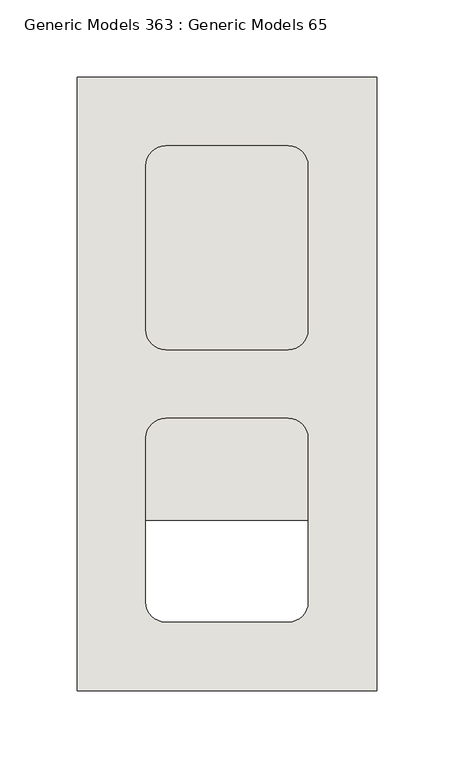
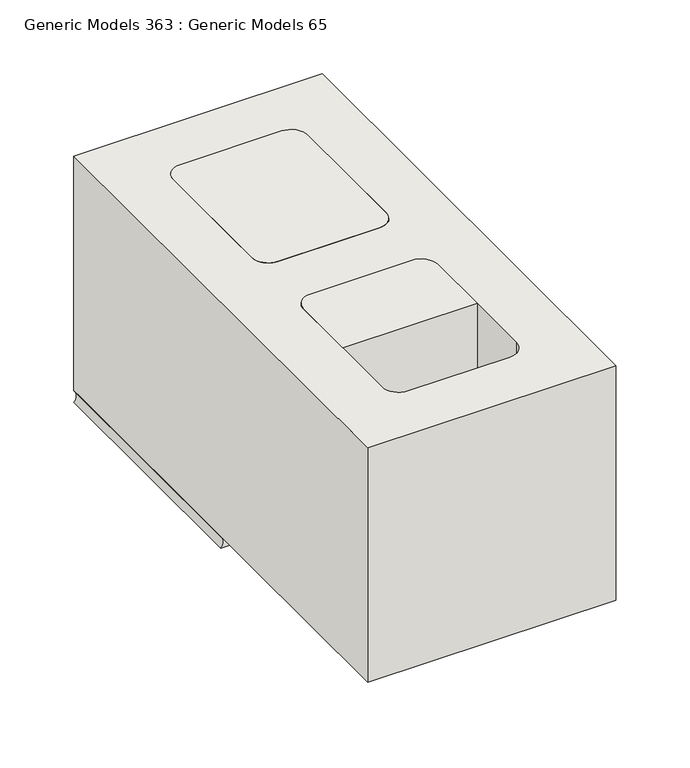
"""IFC4 building model written with IfcOpenShell, lengths in millimetres: wall geometry, Generic Models 363 : Generic Models 65."""

import ifcopenshell
import ifcopenshell.guid

model = None  # the IFC model being written
_history = None  # IfcOwnerHistory: only IFC2X3 demands one
_inside = {}  # id of a spatial element -> (the spatial element, [elements in it])
_under = {}  # id of a project, library or spatial element -> (it, [spatial elements below it])
_declared = {}  # id of a project -> (the project, [libraries it declares])
_typed = {}  # id of a type object -> (the type object, [elements of that type])
_made_of = {}  # id of a material, layer set ... -> (it, [elements and type objects made of it])


def new_model(schema):
    """Start an empty IFC model of exactly this schema.

    Asked for "IFC4X3", IfcOpenShell would pick the latest addendum, in which some entities
    have other attributes; the version numbers below select the first issue.
    IFC2X3 requires an IfcOwnerHistory on every rooted entity: one is made here for all.
    """
    global model, _history
    if schema == "IFC4X3":
        model = ifcopenshell.file(schema_version=(4, 3, 0, 0))
    else:
        model = ifcopenshell.file(schema=schema)
    _inside.clear()
    _under.clear()
    _declared.clear()
    _typed.clear()
    _made_of.clear()
    _history = None
    if model.schema == "IFC2X3":
        org = make("IfcOrganization", Name="unknown")
        user = make(
            "IfcPersonAndOrganization",
            ThePerson=make("IfcPerson", FamilyName="unknown"),
            TheOrganization=org,
        )
        app = make(
            "IfcApplication",
            ApplicationDeveloper=org,
            Version="unknown",
            ApplicationFullName="unknown",
            ApplicationIdentifier="unknown",
        )
        _history = make(
            "IfcOwnerHistory",
            OwningUser=user,
            OwningApplication=app,
            ChangeAction="ADDED",
            CreationDate=0,
        )
    return model


def make(cls, **values):
    """One entity of the class cls with the attributes given. An attribute that is None is left unset."""
    return model.create_entity(
        cls, **{name: value for name, value in values.items() if value is not None}
    )


def rooted(cls, **values):
    """An entity with a GlobalId (a new one), such as an element, a storey or a relation."""
    return make(cls, GlobalId=ifcopenshell.guid.new(), OwnerHistory=_history, **values)


def si_unit(unit_type, name, prefix=None):
    """IfcSIUnit, for example si_unit("LENGTHUNIT", "METRE", prefix="MILLI")."""
    return make("IfcSIUnit", UnitType=unit_type, Prefix=prefix, Name=name)


def assignment(units):
    """IfcUnitAssignment: the units of a project."""
    return None if units is None else make("IfcUnitAssignment", Units=units)


def point(xyz):
    """IfcCartesianPoint."""
    return None if xyz is None else make("IfcCartesianPoint", Coordinates=xyz)


def direction(xyz):
    """IfcDirection."""
    return None if xyz is None else make("IfcDirection", DirectionRatios=xyz)


def frame(location, z_axis=None, x_axis=None):
    """IfcAxis2Placement3D, a coordinate frame: its origin and axes. An axis left out is left unset."""
    return make(
        "IfcAxis2Placement3D",
        Location=point(location),
        Axis=direction(z_axis),
        RefDirection=direction(x_axis),
    )


def frame_2d(location, x_axis=None):
    """IfcAxis2Placement2D, a coordinate frame in the plane: its origin and x axis."""
    return make(
        "IfcAxis2Placement2D", Location=point(location), RefDirection=direction(x_axis)
    )


def origin():
    """The frame at (0, 0, 0) with its axes left unset."""
    return frame((0.0, 0.0, 0.0))


def place(relative_to, where):
    """IfcLocalPlacement: puts the frame where relative to a parent placement (None: the world)."""
    return make(
        "IfcLocalPlacement", PlacementRelTo=relative_to, RelativePlacement=where
    )


def context(
    kind, dimensions, precision=None, world=None, true_north=None, identifier=None
):
    """IfcGeometricRepresentationContext, for example the 3D "Model" context."""
    return make(
        "IfcGeometricRepresentationContext",
        ContextIdentifier=identifier,
        ContextType=kind,
        CoordinateSpaceDimension=dimensions,
        Precision=precision,
        WorldCoordinateSystem=world,
        TrueNorth=true_north,
    )


def project(units=None, contexts=None):
    """IfcProject with its units and contexts."""
    return rooted(
        "IfcProject",
        Name="project",
        RepresentationContexts=contexts,
        UnitsInContext=assignment(units),
    )


def spatial(cls, under=None, at=None, **own):
    """A site, building, storey or space (cls), placed at a placement, below another one or the project."""
    s = rooted(cls, ObjectPlacement=at, **own)
    if under is not None:
        _under.setdefault(under.id(), (under, []))[1].append(s)
    return s


def polyline(points):
    """IfcPolyline through the points."""
    return make("IfcPolyline", Points=[point(p) for p in points])


def circle_curve(where, radius):
    """IfcCircle in the frame where."""
    return make("IfcCircle", Position=where, Radius=radius)


def trimmed(basis, trim1, trim2, sense, master):
    """IfcTrimmedCurve: the piece of a basis curve between two trims."""
    return make(
        "IfcTrimmedCurve",
        BasisCurve=basis,
        Trim1=trim1,
        Trim2=trim2,
        SenseAgreement=sense,
        MasterRepresentation=master,
    )


def segment(curve, same_sense, transition):
    """IfcCompositeCurveSegment."""
    return make(
        "IfcCompositeCurveSegment",
        Transition=transition,
        SameSense=same_sense,
        ParentCurve=curve,
    )


def composite_curve(segments, self_intersect=None):
    """IfcCompositeCurve: segments joined end to end."""
    return make("IfcCompositeCurve", Segments=segments, SelfIntersect=self_intersect)


def outline(outer, holes=None, kind="AREA"):
    """IfcArbitraryClosedProfileDef: a profile drawn as a closed curve; with holes, ...WithVoids."""
    if holes is None:
        return make("IfcArbitraryClosedProfileDef", ProfileType=kind, OuterCurve=outer)
    return make(
        "IfcArbitraryProfileDefWithVoids",
        ProfileType=kind,
        OuterCurve=outer,
        InnerCurves=holes,
    )


def extrude(swept, where, along, depth):
    """IfcExtrudedAreaSolid: the profile swept, set in the frame where, extruded along a direction by depth."""
    return make(
        "IfcExtrudedAreaSolid",
        SweptArea=swept,
        Position=where,
        ExtrudedDirection=direction(along),
        Depth=depth,
    )


def shape(context_of_items, identifier, shape_type, items):
    """IfcShapeRepresentation: the items that make up one representation, for example the "Body"."""
    return make(
        "IfcShapeRepresentation",
        ContextOfItems=context_of_items,
        RepresentationIdentifier=identifier,
        RepresentationType=shape_type,
        Items=items,
    )


def source(mapping_origin, context_of_items, identifier, shape_type, items):
    """IfcRepresentationMap: a shape defined once, which mapped items show again and again."""
    return make(
        "IfcRepresentationMap",
        MappingOrigin=mapping_origin,
        MappedRepresentation=shape(context_of_items, identifier, shape_type, items),
    )


def transform(
    local_origin,
    x_axis=None,
    y_axis=None,
    z_axis=None,
    scale=None,
    scale2=None,
    scale3=None,
    uniform=True,
):
    """IfcCartesianTransformationOperator3D, or its non-uniform kind. x_axis, y_axis, z_axis: its Axis1, 2, 3."""
    if uniform:
        return make(
            "IfcCartesianTransformationOperator3D",
            Axis1=direction(x_axis),
            Axis2=direction(y_axis),
            LocalOrigin=point(local_origin),
            Scale=scale,
            Axis3=direction(z_axis),
        )
    return make(
        "IfcCartesianTransformationOperator3DnonUniform",
        Axis1=direction(x_axis),
        Axis2=direction(y_axis),
        LocalOrigin=point(local_origin),
        Scale=scale,
        Axis3=direction(z_axis),
        Scale2=scale2,
        Scale3=scale3,
    )


def mapped(mapping_source, mapping_target):
    """IfcMappedItem: shows the shape of a source again, moved by a transform."""
    return make(
        "IfcMappedItem", MappingSource=mapping_source, MappingTarget=mapping_target
    )


def made_of(thing, what):
    """Note that an element or type object is made of a material, layer set ...; save() writes the relation."""
    if what is not None:
        _made_of.setdefault(what.id(), (what, []))[1].append(thing)
    return thing


def element(
    cls,
    number,
    at=None,
    inside=None,
    cuts=None,
    type_object=None,
    material=None,
    context=None,
    identifier="Body",
    shape_type=None,
    held_by="IfcProductDefinitionShape",
    body=None,
    shapes=None,
    **own,
):
    """One element of the class cls, such as IfcWall. Its Tag is "e" and its number.

    at: its placement. inside: the storey or other place that contains it. cuts: it is an
    opening in that element (IfcRelVoidsElement). A single representation is given by context,
    identifier, shape_type and body (its items); several are given by shapes. held_by: the class
    of the entity that holds the representations. save() writes the other relations.
    """
    e = rooted(cls, Tag="e%d" % number, ObjectPlacement=at, **own)
    if body is not None:
        shapes = [shape(context, identifier, shape_type, body)]
    if shapes is not None:
        e.Representation = make(held_by, Representations=shapes)
    if inside is not None:
        _inside.setdefault(inside.id(), (inside, []))[1].append(e)
    if cuts is not None:
        rooted(
            "IfcRelVoidsElement", RelatingBuildingElement=cuts, RelatedOpeningElement=e
        )
    if type_object is not None:
        _typed.setdefault(type_object.id(), (type_object, []))[1].append(e)
    return made_of(e, material)


def aggregate(whole, parts):
    """IfcRelAggregates: a whole, such as a stair, and the parts it consists of."""
    return rooted("IfcRelAggregates", RelatingObject=whole, RelatedObjects=parts)


def save(model, path):
    """Write the relations noted so far, then the file.

    IfcRelAggregates (storeys below a building ...), IfcRelContainedInSpatialStructure (elements
    in a storey), IfcRelDefinesByType, IfcRelAssociatesMaterial and IfcRelDeclares: one each for
    every whole, place, type object, material and project.
    """
    for whole, parts in _under.values():
        aggregate(whole, parts)
    for where, things in _inside.values():
        rooted(
            "IfcRelContainedInSpatialStructure",
            RelatedElements=things,
            RelatingStructure=where,
        )
    for kind, things in _typed.values():
        rooted("IfcRelDefinesByType", RelatedObjects=things, RelatingType=kind)
    for what, things in _made_of.values():
        rooted("IfcRelAssociatesMaterial", RelatedObjects=things, RelatingMaterial=what)
    for by, libraries in _declared.values():
        rooted("IfcRelDeclares", RelatingContext=by, RelatedDefinitions=libraries)
    model.write(path)


def plane_surface(at):
    """IfcPlane: the flat surface through the origin of the frame at, square to its z axis."""
    return make("IfcPlane", Position=at)


def revolved_surface(curve, axis_point, axis_direction):
    """IfcSurfaceOfRevolution: the curve turned about the line through axis_point along axis_direction."""
    return make(
        "IfcSurfaceOfRevolution",
        SweptCurve=make("IfcArbitraryOpenProfileDef", ProfileType="CURVE", Curve=curve),
        AxisPosition=make("IfcAxis1Placement", Location=point(axis_point), Axis=direction(axis_direction)),
    )


def advanced_brep(points, edges, surfaces, faces):
    """IfcAdvancedBrep: a solid bounded by faces that lie on surfaces and meet in shared edges.

    An edge is (start, end): straight between two places in points (the first is 0);
    or (start, end, curve); or (start, end, curve, False) where it runs against its curve.
    A face is (place in surfaces, loops), or (place, loops, False) where it looks against
    its surface's normal. A loop lists edges by number (the first is 1), with a minus sign
    where the edge is run from its end to its start. The first loop is the outer one.
    """
    corners = [point(p) for p in points]
    vertices = [make("IfcVertexPoint", VertexGeometry=c) for c in corners]
    made = []
    for start, end, *more in edges:
        made.append(
            make(
                "IfcEdgeCurve",
                EdgeStart=vertices[start],
                EdgeEnd=vertices[end],
                EdgeGeometry=more[0] if more else make("IfcPolyline", Points=[corners[start], corners[end]]),
                SameSense=more[1] if len(more) > 1 else True,
            )
        )
    hull = []
    for where, loops, *sense in faces:
        bounds = []
        for j, loop in enumerate(loops):
            ring = [make("IfcOrientedEdge", EdgeElement=made[abs(k) - 1], Orientation=k > 0) for k in loop]
            bounds.append(
                make(
                    "IfcFaceOuterBound" if j == 0 else "IfcFaceBound",
                    Bound=make("IfcEdgeLoop", EdgeList=ring),
                    Orientation=True,
                )
            )
        hull.append(make("IfcAdvancedFace", Bounds=bounds, FaceSurface=surfaces[where], SameSense=sense[0] if sense else True))
    return make("IfcAdvancedBrep", Outer=make("IfcClosedShell", CfsFaces=hull))


def generic_models_363_generic_models_65_5e5dd987(model_context):
    return source(origin(), model_context, "Body", "SolidModel", [
        advanced_brep(
        [(430198.2125, 503.2375, 1228.725), (430004.5375, 503.2375, 1228.725), (430004.5375, 503.2375, 1219.2), (430198.2125, 503.2375, 1219.2), (430198.2125, 701.675, 1228.725), (430198.2125, 701.675, 1219.2), (430004.5375, 701.675, 1219.2), (430004.5375, 701.675, 1228.725), (430153.7625, 538.1625, 1228.725), (430141.0625, 525.4625, 1228.725), (430061.6875, 525.4625, 1228.725), (430048.9875, 538.1625, 1228.725), (430048.9875, 644.525, 1228.725), (430061.6875, 657.225, 1228.725), (430141.0625, 657.225, 1228.725), (430153.7625, 644.525, 1228.725), (430141.0625, 525.4625, 1219.2), (430153.7625, 538.1625, 1219.2), (430061.6875, 525.4625, 1219.2), (430048.9875, 538.1625, 1219.2), (430048.9875, 644.525, 1219.2), (430061.6875, 657.225, 1219.2), (430141.0625, 657.225, 1219.2), (430153.7625, 644.525, 1219.2)],
        [
            (0, 1),
            (1, 2, circle_curve(frame((429999.6545028, 503.2375, 1223.9625), z_axis=(0.0, 1.0, 0.0), x_axis=(1.0, 0.0, 0.0)), 6.8209287)),
            (2, 3),
            (3, 0, circle_curve(frame((430203.0954972, 503.2375, 1223.9625), z_axis=(0.0, 1.0, 0.0), x_axis=(-1.0, 0.0, 0.0)), 6.8209287)),
            (4, 5, circle_curve(frame((430203.0954972, 701.675, 1223.9625), z_axis=(0.0, -1.0, 0.0), x_axis=(-1.0, 0.0, 0.0)), 6.8209287)),
            (5, 6),
            (6, 7, circle_curve(frame((429999.6545028, 701.675, 1223.9625), z_axis=(0.0, -1.0, 0.0), x_axis=(1.0, 0.0, 0.0)), 6.8209287)),
            (7, 4),
            (0, 4),
            (7, 1),
            (8, 9, circle_curve(frame((430141.0625, 538.1625, 1228.725), z_axis=(0.0, 0.0, -1.0), x_axis=(-1.0, 0.0, 0.0)), 12.7)),
            (9, 10),
            (10, 11, circle_curve(frame((430061.6875, 538.1625, 1228.725), z_axis=(0.0, 0.0, -1.0), x_axis=(-1.0, 0.0, 0.0)), 12.7)),
            (11, 12),
            (12, 13, circle_curve(frame((430061.6875, 644.525, 1228.725), z_axis=(0.0, 0.0, -1.0), x_axis=(-1.0, 0.0, 0.0)), 12.7)),
            (13, 14),
            (14, 15, circle_curve(frame((430141.0625, 644.525, 1228.725), z_axis=(0.0, 0.0, -1.0), x_axis=(-1.0, 0.0, 0.0)), 12.7)),
            (15, 8),
            (16, 9),
            (8, 17),
            (17, 16, circle_curve(frame((430141.0625, 538.1625, 1219.2), z_axis=(0.0, 0.0, -1.0), x_axis=(-1.0, 0.0, 0.0)), 12.7)),
            (16, 18),
            (18, 10),
            (18, 19, circle_curve(frame((430061.6875, 538.1625, 1219.2), z_axis=(0.0, 0.0, -1.0), x_axis=(-1.0, 0.0, 0.0)), 12.7)),
            (19, 11),
            (19, 20),
            (20, 12),
            (20, 21, circle_curve(frame((430061.6875, 644.525, 1219.2), z_axis=(0.0, 0.0, -1.0), x_axis=(-1.0, 0.0, 0.0)), 12.7)),
            (21, 13),
            (21, 22),
            (22, 14),
            (22, 23, circle_curve(frame((430141.0625, 644.525, 1219.2), z_axis=(0.0, 0.0, -1.0), x_axis=(-1.0, 0.0, 0.0)), 12.7)),
            (23, 15),
            (23, 17),
            (6, 2),
            (5, 3),
        ],
        [
            plane_surface(frame((430101.375, 503.2375, 1229.121875), z_axis=(0.0, -1.0, 0.0), x_axis=(0.0, 0.0, 1.0))),
            plane_surface(frame((430101.375, 701.675, 1229.121875), z_axis=(0.0, 1.0, 0.0), x_axis=(0.0, 0.0, 1.0))),
            plane_surface(frame((430198.2125, 503.2375, 1228.725), z_axis=(0.0, 0.0, 1.0), x_axis=(0.0, 1.0, 0.0))),
            revolved_surface(polyline([(430128.3625, 538.1625, 1228.725), (430128.3625, 538.1625, 1219.2)]), (430141.0625, 538.1625, 1412.875), (0.0, 0.0, 1.0)),
            plane_surface(frame((430061.6875, 525.4625, 1412.875), z_axis=(0.0, 1.0, 0.0), x_axis=(0.0, 0.0, -1.0))),
            revolved_surface(polyline([(430048.9875, 538.1625, 1228.725), (430048.9875, 538.1625, 1219.2)]), (430061.6875, 538.1625, 1412.875), (0.0, 0.0, 1.0)),
            plane_surface(frame((430048.9875, 644.525, 1412.875), z_axis=(1.0, 0.0, 0.0), x_axis=(0.0, 0.0, -1.0))),
            revolved_surface(polyline([(430048.9875, 644.525, 1228.725), (430048.9875, 644.525, 1219.2)]), (430061.6875, 644.525, 1412.875), (0.0, 0.0, 1.0)),
            plane_surface(frame((430141.0625, 657.225, 1412.875), z_axis=(0.0, -1.0, 0.0), x_axis=(0.0, 0.0, -1.0))),
            revolved_surface(polyline([(430128.3625, 644.525, 1228.725), (430128.3625, 644.525, 1219.2)]), (430141.0625, 644.525, 1412.875), (0.0, 0.0, 1.0)),
            plane_surface(frame((430153.7625, 538.1625, 1412.875), z_axis=(-1.0, 0.0, 0.0), x_axis=(0.0, 0.0, -1.0))),
            revolved_surface(polyline([(430006.4754315, 701.675, 1223.9625), (430006.4754315, 503.2375, 1223.9625)]), (429999.6545028, 503.2375, 1223.9625), (0.0, 1.0, 0.0)),
            plane_surface(frame((430004.5375, 503.2375, 1219.2), z_axis=(0.0, 0.0, -1.0), x_axis=(0.0, 1.0, 0.0))),
            revolved_surface(polyline([(430196.2745685, 701.675, 1223.9625), (430196.2745685, 503.2375, 1223.9625)]), (430203.0954972, 503.2375, 1223.9625), (0.0, 1.0, 0.0)),
        ],
        [
            (0, [[1, 2, 3, 4]]),
            (1, [[5, 6, 7, 8]]),
            (2, [[-1, 9, -8, 10], [11, 12, 13, 14, 15, 16, 17, 18]]),
            (3, [[19, -11, 20, 21]]),
            (4, [[-19, 22, 23, -12]]),
            (5, [[-23, 24, 25, -13]]),
            (6, [[-25, 26, 27, -14]]),
            (7, [[-27, 28, 29, -15]]),
            (8, [[-29, 30, 31, -16]]),
            (9, [[-31, 32, 33, -17]]),
            (10, [[-33, 34, -20, -18]]),
            (11, [[-2, -10, -7, 35]]),
            (12, [[-3, -35, -6, 36], [-21, -34, -32, -30, -28, -26, -24, -22]]),
            (13, [[-4, -36, -5, -9]]),
        ],
    ),
        extrude(outline(composite_curve([segment(trimmed(circle_curve(frame_2d((430141.0625, 538.1625)), 12.7), [point((430153.7625, 538.1625))], [point((430141.0625, 525.4625))], False, "CARTESIAN"), True, "CONTINUOUS"), segment(polyline([(430141.0625, 525.4625), (430061.6875, 525.4625)]), True, "CONTINUOUS"), segment(trimmed(circle_curve(frame_2d((430061.6875, 538.1625)), 12.7), [point((430061.6875, 525.4625))], [point((430048.9875, 538.1625))], False, "CARTESIAN"), True, "CONTINUOUS"), segment(polyline([(430048.9875, 538.1625), (430048.9875, 644.525)]), True, "CONTINUOUS"), segment(trimmed(circle_curve(frame_2d((430061.6875, 644.525)), 12.7), [point((430048.9875, 644.525))], [point((430061.6875, 657.225))], False, "CARTESIAN"), True, "CONTINUOUS"), segment(polyline([(430061.6875, 657.225), (430141.0625, 657.225)]), True, "CONTINUOUS"), segment(trimmed(circle_curve(frame_2d((430141.0625, 644.525)), 12.7), [point((430141.0625, 657.225))], [point((430153.7625, 644.525))], False, "CARTESIAN"), True, "CONTINUOUS"), segment(polyline([(430153.7625, 644.525), (430153.7625, 538.1625)]), True, "CONTINUOUS")], self_intersect=False)), frame((0.0, 0.0, 1219.2), z_axis=(0.0, 0.0, 1.0), x_axis=(1.0, 0.0, 0.0)), (0.0, 0.0, 1.0), 203.2),
        extrude(outline(composite_curve([segment(trimmed(circle_curve(frame_2d((430061.6875, 468.3125)), 12.7), [point((430048.9875, 468.3125))], [point((430061.6875, 481.0125))], False, "CARTESIAN"), True, "CONTINUOUS"), segment(polyline([(430061.6875, 481.0125), (430141.0625, 481.0125)]), True, "CONTINUOUS"), segment(trimmed(circle_curve(frame_2d((430141.0625, 468.3125)), 12.7), [point((430141.0625, 481.0125))], [point((430153.7625, 468.3125))], False, "CARTESIAN"), True, "CONTINUOUS"), segment(polyline([(430153.7625, 468.3125), (430153.7625, 415.13125), (430048.9875, 415.13125), (430048.9875, 468.3125)]), True, "CONTINUOUS")], self_intersect=False)), frame((0.0, 0.0, 1219.2), z_axis=(0.0, 0.0, 1.0), x_axis=(1.0, 0.0, 0.0)), (0.0, 0.0, 1.0), 203.2),
        extrude(outline(polyline([(430198.2125, 304.8), (430004.5375, 304.8), (430004.5375, 701.675), (430198.2125, 701.675), (430198.2125, 304.8)]), holes=[composite_curve([segment(polyline([(430153.7625, 538.1625), (430153.7625, 644.525)]), True, "CONTINUOUS"), segment(trimmed(circle_curve(frame_2d((430141.0625, 644.525)), 12.7), [point((430153.7625, 644.525))], [point((430141.0625, 657.225))], True, "CARTESIAN"), True, "CONTINUOUS"), segment(polyline([(430141.0625, 657.225), (430061.6875, 657.225)]), True, "CONTINUOUS"), segment(trimmed(circle_curve(frame_2d((430061.6875, 644.525)), 12.7), [point((430061.6875, 657.225))], [point((430048.9875, 644.525))], True, "CARTESIAN"), True, "CONTINUOUS"), segment(polyline([(430048.9875, 644.525), (430048.9875, 538.1625)]), True, "CONTINUOUS"), segment(trimmed(circle_curve(frame_2d((430061.6875, 538.1625)), 12.7), [point((430048.9875, 538.1625))], [point((430061.6875, 525.4625))], True, "CARTESIAN"), True, "CONTINUOUS"), segment(polyline([(430061.6875, 525.4625), (430141.0625, 525.4625)]), True, "CONTINUOUS"), segment(trimmed(circle_curve(frame_2d((430141.0625, 538.1625)), 12.7), [point((430141.0625, 525.4625))], [point((430153.7625, 538.1625))], True, "CARTESIAN"), True, "CONTINUOUS")], self_intersect=False), composite_curve([segment(polyline([(430048.9875, 468.3125), (430048.9875, 361.95)]), True, "CONTINUOUS"), segment(trimmed(circle_curve(frame_2d((430061.6875, 361.95)), 12.7), [point((430048.9875, 361.95))], [point((430061.6875, 349.25))], True, "CARTESIAN"), True, "CONTINUOUS"), segment(polyline([(430061.6875, 349.25), (430141.0625, 349.25)]), True, "CONTINUOUS"), segment(trimmed(circle_curve(frame_2d((430141.0625, 361.95)), 12.7), [point((430141.0625, 349.25))], [point((430153.7625, 361.95))], True, "CARTESIAN"), True, "CONTINUOUS"), segment(polyline([(430153.7625, 361.95), (430153.7625, 468.3125)]), True, "CONTINUOUS"), segment(trimmed(circle_curve(frame_2d((430141.0625, 468.3125)), 12.7), [point((430153.7625, 468.3125))], [point((430141.0625, 481.0125))], True, "CARTESIAN"), True, "CONTINUOUS"), segment(polyline([(430141.0625, 481.0125), (430061.6875, 481.0125)]), True, "CONTINUOUS"), segment(trimmed(circle_curve(frame_2d((430061.6875, 468.3125)), 12.7), [point((430061.6875, 481.0125))], [point((430048.9875, 468.3125))], True, "CARTESIAN"), True, "CONTINUOUS")], self_intersect=False)]), frame((0.0, 0.0, 1228.725), z_axis=(0.0, 0.0, 1.0), x_axis=(1.0, 0.0, 0.0)), (0.0, 0.0, 1.0), 193.675),
    ])


if __name__ == "__main__":
    model = new_model("IFC4")
    model_context = context("Model", 3, world=origin())
    ifc_project = project(units=[si_unit("LENGTHUNIT", "METRE", prefix="MILLI")], contexts=[model_context])
    site = spatial("IfcSite", under=ifc_project)
    building = spatial("IfcBuilding", under=site)
    placement = place(None, origin())
    generic_models_363_generic_models_65_shape = generic_models_363_generic_models_65_5e5dd987(model_context)
    element("IfcWall", 1, ObjectType="Generic Models 363 : Generic Models 65", at=placement, inside=building, context=model_context, shape_type="MappedRepresentation", body=[
        mapped(generic_models_363_generic_models_65_shape, transform((0.0, 0.0, 0.0), x_axis=(1.0, 0.0, 0.0), y_axis=(0.0, 1.0, 0.0), z_axis=(0.0, 0.0, 1.0))),
    ])
    save(model, "model.ifc")

# Revit data of these elements
# Element 1 (IfcWall, "Generic Models 363 : Generic Models 65")
#   Materials on its faces: "CMU (SEE 'WALL TAG' FOR SIZE)", "FILL CORE IF APPLICABLE - SEE STRUCTURAL DWGS FOR DETAILS", "MORTAR JOINT"
# Materials
#   "CMU (SEE 'WALL TAG' FOR SIZE)": class "Masonry", colour RGB 203 203 199, transparency 0, Description = "Concrete masonry units", Cost = 0
#   "FILL CORE IF APPLICABLE - SEE STRUCTURAL DWGS FOR DETAILS": class "Generic", colour RGB 170 170 170, transparency 0, Cost = 0
#   "MORTAR JOINT": class "Generic", colour RGB 120 120 120, transparency 0, Cost = 0
